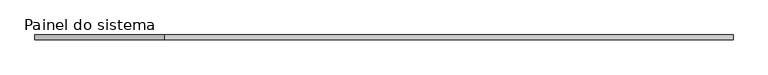
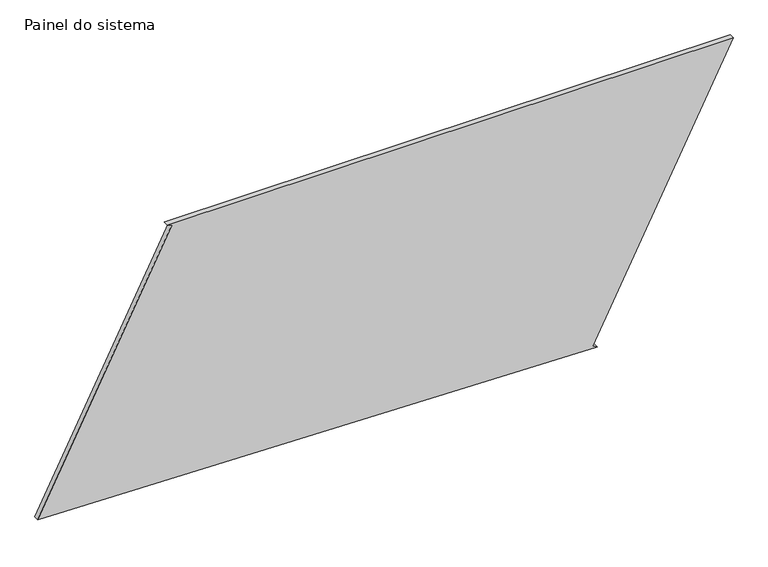
"""IFC4 building model written with IfcOpenShell, lengths in millimetres: plate geometry, Painel do sistema : Envidraçado."""

from ifc_helpers import new_model, si_unit, frame, origin, place, context, project, spatial, polyline, outline, extrude, source, transform, mapped, element, save


def painel_do_sistema_6a82aa62(model_context):
    return source(origin(), model_context, "Body", "SweptSolid", [
        extrude(outline(polyline([(0.0, 1068.1708345), (11.291819, 1045.8662425), (1410.2140359, 1754.0780945), (1410.2140359, -1101.420156), (1398.9222169, -1079.115564), (65.6769784, -1754.0780945), (0.0, 1068.1708345)])), frame((0.0, 24.5, 0.0), z_axis=(0.0, 1.0, 0.0), x_axis=(0.0, 0.0, 1.0)), (0.0, 0.0, 1.0), 25.0),
    ])


if __name__ == "__main__":
    model = new_model("IFC4")
    model_context = context("Model", 3, world=origin())
    ifc_project = project(units=[si_unit("LENGTHUNIT", "METRE", prefix="MILLI")], contexts=[model_context])
    site = spatial("IfcSite", under=ifc_project)
    building = spatial("IfcBuilding", under=site)
    placement = place(None, origin())
    painel_do_sistema_shape = painel_do_sistema_6a82aa62(model_context)
    element("IfcPlate", 1, ObjectType="Painel do sistema : Envidraçado", at=placement, inside=building, context=model_context, shape_type="MappedRepresentation", body=[
        mapped(painel_do_sistema_shape, transform((0.0, 0.0, 0.0), x_axis=(1.0, 0.0, 0.0), y_axis=(0.0, 1.0, 0.0), z_axis=(0.0, 0.0, 1.0))),
    ])
    save(model, "model.ifc")

# Revit data of these elements
# Type "Painel do sistema : Envidraçado"
#   Construction Type Id = "GSP4R"
#   Analytic Construction = "Vidraça única Pilkington 1/8 pol"
#   Visual Light Transmittance = 0.9
#   Solar Heat Gain Coefficient = 0.86
#   Heat Transfer Coefficient (U) = 6.7069 W/(m²·K)
# Element 1 (IfcPlate, "Painel do sistema : Envidraçado")
#   Materials on its faces: "Vidro"
# Materials
#   "Vidro": class "Vidro", colour RGB 0 128 192, transparency 0.9, Description = "Vidro de sílica", Cost = 0
